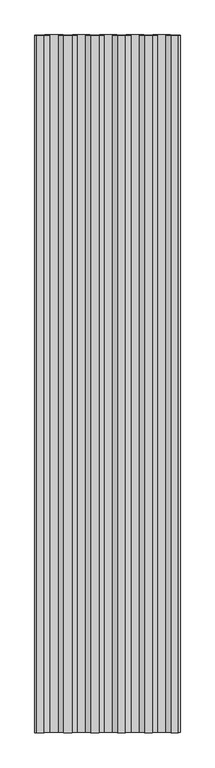
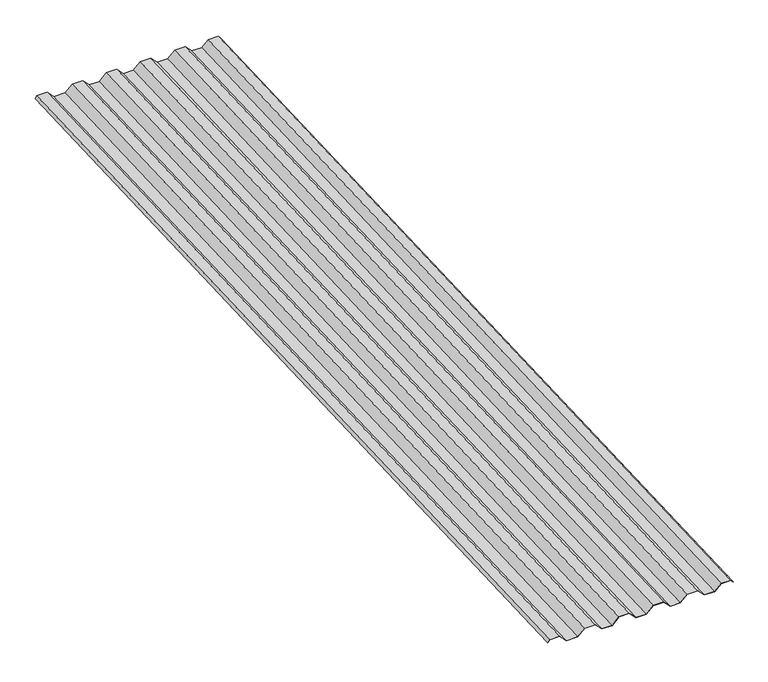
"""IFC4 building model written with IfcOpenShell, lengths in millimetres: proxy geometry, Generic Models 2:Generic Models 2:310765:Generic Models 2:310765 : Generic Models 2:Generic Models 2:310765:4 : Generic Models 2:Generic Models 2:310765:Generic Models 2:310765 : Generic Models 2:Generic Models 2:310765:300385."""

from ifc_helpers import new_model, si_unit, frame, origin, place, context, project, spatial, polyline, outline, extrude, source, transform, mapped, element, save


def generic_models_4eabba17(model_context):
    return source(origin(), model_context, "Body", "SweptSolid", [
        extrude(outline(polyline([(17.6742821, 0.0), (52.9537246, -39.0060166), (49.8838639, -87.1303114), (86.4475987, -127.5562804), (138.3729183, -129.3511562), (175.9688772, -170.9183834), (172.5580906, -222.7626398), (209.1218253, -263.1886088), (261.047145, -264.9834846), (298.6431039, -306.5507118), (295.2323172, -358.3949682), (331.796052, -398.8209372), (383.7213716, -400.615813), (421.3173306, -442.1830402), (417.9065439, -494.0272966), (454.4702787, -534.4532656), (506.3955983, -536.2481414), (543.9915572, -577.8153686), (540.5807706, -629.659625), (581.4040271, -674.7950498), (633.3293468, -676.5899257), (670.4091936, -717.5865237), (666.8444039, -733.1864045), (666.0706003, -733.0095796), (669.5433408, -717.8125156), (632.966081, -677.3715929), (581.0407615, -675.5767171), (539.7666724, -629.9428382), (543.1774589, -578.0985817), (506.0323326, -537.0298086), (454.107013, -535.2349329), (417.0924457, -494.3105098), (420.5032323, -442.4662533), (383.3581059, -401.3974802), (331.4327863, -399.6026045), (294.418219, -358.6781814), (297.8290056, -306.8339249), (260.6838792, -265.7651518), (208.7585597, -263.9702761), (171.7439923, -223.045853), (175.1547789, -171.2015965), (138.0096525, -130.1328234), (86.084333, -128.3379477), (49.0703903, -87.4142152), (52.1402509, -39.2899204), (17.3219447, -0.79375), (-0.0398189, -0.79375), (0.0, 0.0), (17.6742821, 0.0)])), frame((601688.2867239, -541218.9478993, 9908.3379163), z_axis=(0.0, 0.9991330730923567, 0.04163054471206784), x_axis=(-0.6707908283133093, -0.03087515153093964, 0.741003636744575)), (0.0, 0.0, 1.0), 4754.1272401),
    ])


if __name__ == "__main__":
    model = new_model("IFC4")
    model_context = context("Model", 3, world=origin())
    ifc_project = project(units=[si_unit("LENGTHUNIT", "METRE", prefix="MILLI")], contexts=[model_context])
    site = spatial("IfcSite", under=ifc_project)
    building = spatial("IfcBuilding", under=site)
    placement = place(None, origin())
    generic_models_shape = generic_models_4eabba17(model_context)
    element("IfcBuildingElementProxy", 1, Name="Generic Models 2:Generic Models 2:310765:Generic Models 2:310765 : Generic Models 2:Generic Models 2:310765:4 : Generic Models 2:Generic Models 2:310765:Generic Models 2:310765 : Generic Models 2:Generic Models 2:310765:300385", ObjectType="Generic Models 2:Generic Models 2:310765:Generic Models 2:310765 : Generic Models 2:Generic Models 2:310765:4 : Generic Models 2:Generic Models 2:310765:Generic Models 2:310765 : Generic Models 2:Generic Models 2:310765:300385", at=placement, inside=building, context=model_context, shape_type="MappedRepresentation", body=[
        mapped(generic_models_shape, transform((0.0, 0.0, 0.0), x_axis=(1.0, 0.0, 0.0), y_axis=(0.0, 1.0, 0.0), z_axis=(0.0, 0.0, 1.0))),
    ])
    save(model, "model.ifc")

# Revit data of these elements
# Type "Generic Models 2:Generic Models 2:310765:Generic Models 2:310765 : Generic Models 2:Generic Models 2:310765:4 : Generic Models 2:Generic Models 2:310765:Generic Models 2:310765 : Generic Models 2:Generic Models 2:310765:300385"
#   NameOverride = "Generic Models 2:Generic Models 2:310765:Generic Models 2:310765 : Generic Models 2:Generic Models 2:310765:300385"
#   ObjectTypeOverride = "Generic Models 2:310765 : Generic Models 2:Generic Models 2:310765"
#   Reference = "Generic Models 2"
#   Tag = "300385"
# Element 1 (IfcBuildingElementProxy, "Generic Models 2:Generic Models 2:310765:Generic Models 2:310765 : Generic Models 2:Generic Models 2:310765:4 : Generic Models 2:Generic Models 2:310765:Generic Models 2:310765 : Generic Models 2:Generic Models 2:310765:300385")
#   Materials on its faces: "THERMAL BROKEN ALUMINUM STOREFRONT FOR POLYCARBONATE"
# Materials
#   "THERMAL BROKEN ALUMINUM STOREFRONT FOR POLYCARBONATE": class "Unassigned", colour RGB 244 244 244, transparency 0, Keynote = "M07611300.01", Cost = 0
